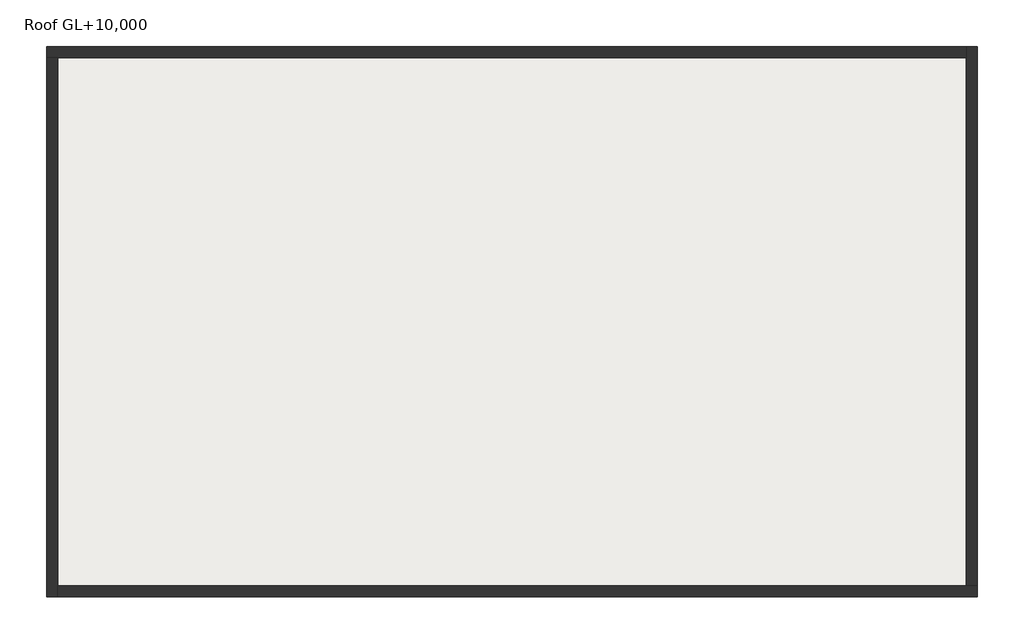
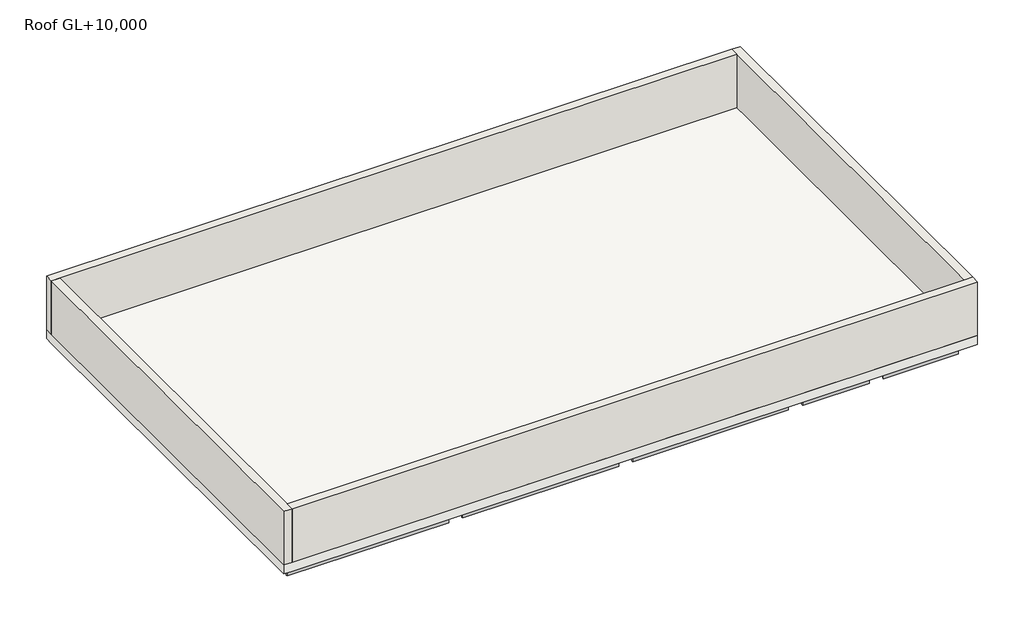
# One storey: 25 beams, 4 walls, 1 roof.
"""IFC4 building model written with IfcOpenShell, lengths in millimetres."""

from ifc_helpers import new_model, si_unit, frame, origin, place, context, project, spatial, polyline, outline, extrude, faceted_brep, element, save

model = new_model("IFC4")

# Units and contexts
model_context = context("Model", 3, world=origin())
ifc_project = project(units=[si_unit("LENGTHUNIT", "METRE", prefix="MILLI")], contexts=[model_context])

# Site, building, storey
site = spatial("IfcSite", under=ifc_project)
building = spatial("IfcBuilding", under=site)
storey = spatial("IfcBuildingStorey", under=building, Name="Roof GL+10,000", Elevation=10000.0)

# Beams
placement = place(None, origin())
element("IfcBeam", 1, ObjectType="RC Beam_Rectangular : 350 x 700mm", at=placement, inside=storey, context=model_context, shape_type="SweptSolid", body=[
    extrude(outline(polyline([(-18645.7273237, 1485.9763125), (-18595.7273237, 1485.9763125), (-18595.7273237, -4314.0236875), (-18645.7273237, -4314.0236875), (-18645.7273237, 1485.9763125)])), frame((0.0, 0.0, 9300.0), z_axis=(0.0, 0.0, 1.0), x_axis=(1.0, 0.0, 0.0)), (0.0, 0.0, 1.0), 367.0),
])
element("IfcBeam", 2, ObjectType="RC Beam_Rectangular : 350 x 700mm", at=placement, inside=storey, context=model_context, shape_type="SweptSolid", body=[
    extrude(outline(polyline([(-18645.7273237, 9185.9763125), (-18595.7273237, 9185.9763125), (-18595.7273237, 1985.9763125), (-18645.7273237, 1985.9763125), (-18645.7273237, 9185.9763125)])), frame((0.0, 0.0, 9300.0), z_axis=(0.0, 0.0, 1.0), x_axis=(1.0, 0.0, 0.0)), (0.0, 0.0, 1.0), 367.0),
])
element("IfcBeam", 3, ObjectType="RC Beam_Rectangular : 350 x 700mm", at=placement, inside=storey, context=model_context, shape_type="SweptSolid", body=[
    extrude(outline(polyline([(-12545.7273237, 1485.9763125), (-12520.7273237, 1485.9763125), (-12520.7273237, -4314.0236875), (-12545.7273237, -4314.0236875), (-12545.7273237, 1485.9763125)])), frame((0.0, 0.0, 9300.0), z_axis=(0.0, 0.0, 1.0), x_axis=(1.0, 0.0, 0.0)), (0.0, 0.0, 1.0), 367.0),
    extrude(outline(polyline([(-12870.7273237, 1485.9763125), (-12845.7273237, 1485.9763125), (-12845.7273237, -4314.0236875), (-12870.7273237, -4314.0236875), (-12870.7273237, 1485.9763125)])), frame((0.0, 0.0, 9300.0), z_axis=(0.0, 0.0, 1.0), x_axis=(1.0, 0.0, 0.0)), (0.0, 0.0, 1.0), 367.0),
])
element("IfcBeam", 4, ObjectType="RC Beam_Rectangular : 350 x 700mm", at=placement, inside=storey, context=model_context, shape_type="Brep", body=[
    faceted_brep([(-12520.7273237, 5725.9613486, 9667.0), (-12520.7273237, 5725.9613486, 9300.0), (-12520.7273237, 9185.9763125, 9300.0), (-12520.7273237, 9185.9763125, 9667.0), (-12545.7273237, 5725.9613486, 9300.0), (-12545.7273237, 9185.9763125, 9300.0), (-12545.7273237, 5725.9613486, 9667.0), (-12545.7273237, 9185.9763125, 9667.0)], [[[0, 1, 2, 3]], [[1, 4, 5, 2]], [[4, 6, 7, 5]], [[1, 0, 6, 4]], [[6, 0, 3, 7]], [[2, 5, 7, 3]]]),
    faceted_brep([(-12870.7273237, 9185.9763125, 9667.0), (-12870.7273237, 9185.9763125, 9300.0), (-12870.7273237, 1985.9763125, 9300.0), (-12870.7273237, 1985.9763125, 9667.0), (-12520.7273237, 5425.9613486, 9667.0), (-12545.7273237, 5425.9613486, 9667.0), (-12845.7273237, 5425.9613486, 9667.0), (-12845.7273237, 9185.9763125, 9667.0), (-12520.7273237, 1985.9763125, 9667.0), (-12845.7273237, 5425.9613486, 9300.0), (-12845.7273237, 9185.9763125, 9300.0), (-12520.7273237, 5425.9613486, 9300.0), (-12520.7273237, 1985.9763125, 9300.0)], [[[0, 1, 2, 3]], [[4, 5, 6, 7, 0, 3, 8]], [[6, 9, 10, 7]], [[9, 6, 5, 4, 11]], [[11, 4, 8, 12]], [[9, 11, 12, 2, 1, 10]], [[1, 0, 7, 10]], [[3, 2, 12, 8]]]),
])
element("IfcBeam", 5, ObjectType="RC Beam_Rectangular : 350 x 700mm", at=placement, inside=storey, context=model_context, shape_type="SweptSolid", body=[
    extrude(outline(polyline([(-6545.7273237, 1485.9763125), (-6520.7273237, 1485.9763125), (-6520.7273237, -4314.0236875), (-6545.7273237, -4314.0236875), (-6545.7273237, 1485.9763125)])), frame((0.0, 0.0, 9300.0), z_axis=(0.0, 0.0, 1.0), x_axis=(1.0, 0.0, 0.0)), (0.0, 0.0, 1.0), 367.0),
    extrude(outline(polyline([(-6870.7273237, 1485.9763125), (-6845.7273237, 1485.9763125), (-6845.7273237, -4314.0236875), (-6870.7273237, -4314.0236875), (-6870.7273237, 1485.9763125)])), frame((0.0, 0.0, 9300.0), z_axis=(0.0, 0.0, 1.0), x_axis=(1.0, 0.0, 0.0)), (0.0, 0.0, 1.0), 367.0),
])
element("IfcBeam", 6, ObjectType="RC Beam_Rectangular : 350 x 700mm", at=placement, inside=storey, context=model_context, shape_type="SweptSolid", body=[
    extrude(outline(polyline([(-6545.7273237, 9185.9763125), (-6520.7273237, 9185.9763125), (-6520.7273237, 1985.9763125), (-6545.7273237, 1985.9763125), (-6545.7273237, 9185.9763125)])), frame((0.0, 0.0, 9300.0), z_axis=(0.0, 0.0, 1.0), x_axis=(1.0, 0.0, 0.0)), (0.0, 0.0, 1.0), 367.0),
    extrude(outline(polyline([(-6845.7273237, 5725.9613486), (-6870.7273237, 5725.9613486), (-6870.7273237, 9185.9763125), (-6845.7273237, 9185.9763125), (-6845.7273237, 5725.9613486)])), frame((0.0, 0.0, 9300.0), z_axis=(0.0, 0.0, 1.0), x_axis=(1.0, 0.0, 0.0)), (0.0, 0.0, 1.0), 367.0),
    extrude(outline(polyline([(-6870.7273237, 5425.9613486), (-6845.7273237, 5425.9613486), (-6845.7273237, 1985.9763125), (-6870.7273237, 1985.9763125), (-6870.7273237, 5425.9613486)])), frame((0.0, 0.0, 9300.0), z_axis=(0.0, 0.0, 1.0), x_axis=(1.0, 0.0, 0.0)), (0.0, 0.0, 1.0), 367.0),
])
element("IfcBeam", 7, ObjectType="RC Beam_Rectangular : 350 x 700mm", at=placement, inside=storey, context=model_context, shape_type="SweptSolid", body=[
    extrude(outline(polyline([(-545.7273237, 1485.9763125), (-520.7273237, 1485.9763125), (-520.7273237, -4314.0236875), (-545.7273237, -4314.0236875), (-545.7273237, 1485.9763125)])), frame((0.0, 0.0, 9300.0), z_axis=(0.0, 0.0, 1.0), x_axis=(1.0, 0.0, 0.0)), (0.0, 0.0, 1.0), 367.0),
    extrude(outline(polyline([(-870.7273237, 1485.9763125), (-845.7273237, 1485.9763125), (-845.7273237, -4314.0236875), (-870.7273237, -4314.0236875), (-870.7273237, 1485.9763125)])), frame((0.0, 0.0, 9300.0), z_axis=(0.0, 0.0, 1.0), x_axis=(1.0, 0.0, 0.0)), (0.0, 0.0, 1.0), 367.0),
])
element("IfcBeam", 8, ObjectType="RC Beam_Rectangular : 350 x 700mm", at=placement, inside=storey, context=model_context, shape_type="SweptSolid", body=[
    extrude(outline(polyline([(-870.7273237, 9185.9763125), (-520.7273237, 9185.9763125), (-520.7273237, 1985.9763125), (-870.7273237, 1985.9763125), (-870.7273237, 9185.9763125)])), frame((0.0, 0.0, 9300.0), z_axis=(0.0, 0.0, 1.0), x_axis=(1.0, 0.0, 0.0)), (0.0, 0.0, 1.0), 367.0),
])
element("IfcBeam", 9, ObjectType="RC Beam_Rectangular : 350 x 700mm", at=placement, inside=storey, context=model_context, shape_type="SweptSolid", body=[
    extrude(outline(polyline([(5204.2726763, 1485.9763125), (5254.2726763, 1485.9763125), (5254.2726763, -4314.0236875), (5204.2726763, -4314.0236875), (5204.2726763, 1485.9763125)])), frame((0.0, 0.0, 9300.0), z_axis=(0.0, 0.0, 1.0), x_axis=(1.0, 0.0, 0.0)), (0.0, 0.0, 1.0), 367.0),
])
element("IfcBeam", 10, ObjectType="RC Beam_Rectangular : 350 x 700mm", at=placement, inside=storey, context=model_context, shape_type="SweptSolid", body=[
    extrude(outline(polyline([(5204.2726763, 9185.9763125), (5254.2726763, 9185.9763125), (5254.2726763, 1885.9763125), (5204.2726763, 1885.9763125), (5204.2726763, 9185.9763125)])), frame((0.0, 0.0, 9300.0), z_axis=(0.0, 0.0, 1.0), x_axis=(1.0, 0.0, 0.0)), (0.0, 0.0, 1.0), 367.0),
])
element("IfcBeam", 11, ObjectType="RC Beam_Rectangular : 350 x 700mm", at=placement, inside=storey, context=model_context, shape_type="SweptSolid", body=[
    extrude(outline(polyline([(-18445.7273237, 9335.9763125), (-18445.7273237, 9385.9763125), (-12945.7273237, 9385.9763125), (-12945.7273237, 9335.9763125), (-18445.7273237, 9335.9763125)])), frame((0.0, 0.0, 9300.0), z_axis=(0.0, 0.0, 1.0), x_axis=(1.0, 0.0, 0.0)), (0.0, 0.0, 1.0), 367.0),
])
element("IfcBeam", 12, ObjectType="RC Beam_Rectangular : 350 x 700mm", at=placement, inside=storey, context=model_context, shape_type="SweptSolid", body=[
    extrude(outline(polyline([(-12445.7273237, 9335.9763125), (-12445.7273237, 9385.9763125), (-6945.7273237, 9385.9763125), (-6945.7273237, 9335.9763125), (-12445.7273237, 9335.9763125)])), frame((0.0, 0.0, 9300.0), z_axis=(0.0, 0.0, 1.0), x_axis=(1.0, 0.0, 0.0)), (0.0, 0.0, 1.0), 367.0),
])
element("IfcBeam", 13, ObjectType="RC Beam_Rectangular : 350 x 700mm", at=placement, inside=storey, context=model_context, shape_type="SweptSolid", body=[
    extrude(outline(polyline([(-6445.7273237, 9335.9763125), (-6445.7273237, 9385.9763125), (-945.7273237, 9385.9763125), (-945.7273237, 9335.9763125), (-6445.7273237, 9335.9763125)])), frame((0.0, 0.0, 9300.0), z_axis=(0.0, 0.0, 1.0), x_axis=(1.0, 0.0, 0.0)), (0.0, 0.0, 1.0), 367.0),
])
element("IfcBeam", 14, ObjectType="RC Beam_Rectangular : 350 x 700mm", at=placement, inside=storey, context=model_context, shape_type="SweptSolid", body=[
    extrude(outline(polyline([(-445.7273237, 9385.9763125), (5254.2726763, 9385.9763125), (5254.2726763, 9335.9763125), (-445.7273237, 9335.9763125), (-445.7273237, 9385.9763125)])), frame((0.0, 0.0, 9300.0), z_axis=(0.0, 0.0, 1.0), x_axis=(1.0, 0.0, 0.0)), (0.0, 0.0, 1.0), 367.0),
])
element("IfcBeam", 15, ObjectType="RC Beam_Rectangular : 350 x 700mm", at=placement, inside=storey, context=model_context, shape_type="SweptSolid", body=[
    extrude(outline(polyline([(-18445.7273237, 1560.9763125), (-18445.7273237, 1585.9763125), (-12945.7273237, 1585.9763125), (-12945.7273237, 1560.9763125), (-18445.7273237, 1560.9763125)])), frame((0.0, 0.0, 9300.0), z_axis=(0.0, 0.0, 1.0), x_axis=(1.0, 0.0, 0.0)), (0.0, 0.0, 1.0), 367.0),
    extrude(outline(polyline([(-18445.7273237, 1885.9763125), (-18445.7273237, 1910.9763125), (-12945.7273237, 1910.9763125), (-12945.7273237, 1885.9763125), (-18445.7273237, 1885.9763125)])), frame((0.0, 0.0, 9300.0), z_axis=(0.0, 0.0, 1.0), x_axis=(1.0, 0.0, 0.0)), (0.0, 0.0, 1.0), 367.0),
])
element("IfcBeam", 16, ObjectType="RC Beam_Rectangular : 350 x 700mm", at=placement, inside=storey, context=model_context, shape_type="SweptSolid", body=[
    extrude(outline(polyline([(-12445.7273237, 1560.9763125), (-12445.7273237, 1585.9763125), (-6945.7273237, 1585.9763125), (-6945.7273237, 1560.9763125), (-12445.7273237, 1560.9763125)])), frame((0.0, 0.0, 9300.0), z_axis=(0.0, 0.0, 1.0), x_axis=(1.0, 0.0, 0.0)), (0.0, 0.0, 1.0), 367.0),
    extrude(outline(polyline([(-12445.7273237, 1885.9763125), (-12445.7273237, 1910.9763125), (-6945.7273237, 1910.9763125), (-6945.7273237, 1885.9763125), (-12445.7273237, 1885.9763125)])), frame((0.0, 0.0, 9300.0), z_axis=(0.0, 0.0, 1.0), x_axis=(1.0, 0.0, 0.0)), (0.0, 0.0, 1.0), 367.0),
])
element("IfcBeam", 17, ObjectType="RC Beam_Rectangular : 350 x 700mm", at=placement, inside=storey, context=model_context, shape_type="SweptSolid", body=[
    extrude(outline(polyline([(-6445.7273237, 1560.9763125), (-6445.7273237, 1585.9763125), (-945.7273237, 1585.9763125), (-945.7273237, 1560.9763125), (-6445.7273237, 1560.9763125)])), frame((0.0, 0.0, 9300.0), z_axis=(0.0, 0.0, 1.0), x_axis=(1.0, 0.0, 0.0)), (0.0, 0.0, 1.0), 367.0),
    extrude(outline(polyline([(-6445.7273237, 1885.9763125), (-6445.7273237, 1910.9763125), (-945.7273237, 1910.9763125), (-945.7273237, 1885.9763125), (-6445.7273237, 1885.9763125)])), frame((0.0, 0.0, 9300.0), z_axis=(0.0, 0.0, 1.0), x_axis=(1.0, 0.0, 0.0)), (0.0, 0.0, 1.0), 367.0),
])
element("IfcBeam", 18, ObjectType="RC Beam_Rectangular : 350 x 700mm", at=placement, inside=storey, context=model_context, shape_type="SweptSolid", body=[
    extrude(outline(polyline([(-445.7273237, 1560.9763125), (-445.7273237, 1585.9763125), (1904.2726763, 1585.9763125), (1904.2726763, 1560.9763125), (-445.7273237, 1560.9763125)])), frame((0.0, 0.0, 9300.0), z_axis=(0.0, 0.0, 1.0), x_axis=(1.0, 0.0, 0.0)), (0.0, 0.0, 1.0), 367.0),
    extrude(outline(polyline([(-445.7273237, 1885.9763125), (-445.7273237, 1910.9763125), (1904.2726763, 1910.9763125), (1904.2726763, 1885.9763125), (-445.7273237, 1885.9763125)])), frame((0.0, 0.0, 9300.0), z_axis=(0.0, 0.0, 1.0), x_axis=(1.0, 0.0, 0.0)), (0.0, 0.0, 1.0), 367.0),
])
element("IfcBeam", 19, ObjectType="RC Beam_Rectangular : 350 x 700mm", at=placement, inside=storey, context=model_context, shape_type="SweptSolid", body=[
    extrude(outline(polyline([(5054.2726763, 1585.9763125), (5054.2726763, 1560.9763125), (2404.2726763, 1560.9763125), (2404.2726763, 1585.9763125), (5054.2726763, 1585.9763125)])), frame((0.0, 0.0, 9300.0), z_axis=(0.0, 0.0, 1.0), x_axis=(1.0, 0.0, 0.0)), (0.0, 0.0, 1.0), 367.0),
    extrude(outline(polyline([(5054.2726763, 1910.9763125), (5054.2726763, 1885.9763125), (2404.2726763, 1885.9763125), (2404.2726763, 1910.9763125), (5054.2726763, 1910.9763125)])), frame((0.0, 0.0, 9300.0), z_axis=(0.0, 0.0, 1.0), x_axis=(1.0, 0.0, 0.0)), (0.0, 0.0, 1.0), 367.0),
])
element("IfcBeam", 20, ObjectType="RC Beam_Rectangular : 350 x 700mm", at=placement, inside=storey, context=model_context, shape_type="SweptSolid", body=[
    extrude(outline(polyline([(-12945.7273237, -4514.0236875), (-18645.7273237, -4514.0236875), (-18645.7273237, -4464.0236875), (-12945.7273237, -4464.0236875), (-12945.7273237, -4514.0236875)])), frame((0.0, 0.0, 9300.0), z_axis=(0.0, 0.0, 1.0), x_axis=(1.0, 0.0, 0.0)), (0.0, 0.0, 1.0), 367.0),
])
element("IfcBeam", 21, ObjectType="RC Beam_Rectangular : 350 x 700mm", at=placement, inside=storey, context=model_context, shape_type="SweptSolid", body=[
    extrude(outline(polyline([(-12445.7273237, -4514.0236875), (-12445.7273237, -4464.0236875), (-6945.7273237, -4464.0236875), (-6945.7273237, -4514.0236875), (-12445.7273237, -4514.0236875)])), frame((0.0, 0.0, 9300.0), z_axis=(0.0, 0.0, 1.0), x_axis=(1.0, 0.0, 0.0)), (0.0, 0.0, 1.0), 367.0),
])
element("IfcBeam", 22, ObjectType="RC Beam_Rectangular : 350 x 700mm", at=placement, inside=storey, context=model_context, shape_type="SweptSolid", body=[
    extrude(outline(polyline([(-6445.7273237, -4514.0236875), (-6445.7273237, -4464.0236875), (-945.7273237, -4464.0236875), (-945.7273237, -4514.0236875), (-6445.7273237, -4514.0236875)])), frame((0.0, 0.0, 9300.0), z_axis=(0.0, 0.0, 1.0), x_axis=(1.0, 0.0, 0.0)), (0.0, 0.0, 1.0), 367.0),
])
element("IfcBeam", 23, ObjectType="RC Beam_Rectangular : 350 x 700mm", at=placement, inside=storey, context=model_context, shape_type="SweptSolid", body=[
    extrude(outline(polyline([(-445.7273237, -4514.0236875), (-445.7273237, -4464.0236875), (1904.2726763, -4464.0236875), (1904.2726763, -4514.0236875), (-445.7273237, -4514.0236875)])), frame((0.0, 0.0, 9300.0), z_axis=(0.0, 0.0, 1.0), x_axis=(1.0, 0.0, 0.0)), (0.0, 0.0, 1.0), 367.0),
])
element("IfcBeam", 24, ObjectType="RC Beam_Rectangular : 350 x 700mm", at=placement, inside=storey, context=model_context, shape_type="SweptSolid", body=[
    extrude(outline(polyline([(5054.2726763, -4464.0236875), (5054.2726763, -4514.0236875), (2404.2726763, -4514.0236875), (2404.2726763, -4464.0236875), (5054.2726763, -4464.0236875)])), frame((0.0, 0.0, 9300.0), z_axis=(0.0, 0.0, 1.0), x_axis=(1.0, 0.0, 0.0)), (0.0, 0.0, 1.0), 367.0),
])
element("IfcBeam", 25, ObjectType="RC Beam_Rectangular : 350 x 700mm", at=placement, inside=storey, context=model_context, shape_type="SweptSolid", body=[
    extrude(outline(polyline([(2304.2726763, 1485.9763125), (2329.2726763, 1485.9763125), (2329.2726763, -4314.0236875), (2304.2726763, -4314.0236875), (2304.2726763, 1485.9763125)])), frame((0.0, 0.0, 9300.0), z_axis=(0.0, 0.0, 1.0), x_axis=(1.0, 0.0, 0.0)), (0.0, 0.0, 1.0), 367.0),
    extrude(outline(polyline([(1979.2726763, 1485.9763125), (2004.2726763, 1485.9763125), (2004.2726763, -4314.0236875), (1979.2726763, -4314.0236875), (1979.2726763, 1485.9763125)])), frame((0.0, 0.0, 9300.0), z_axis=(0.0, 0.0, 1.0), x_axis=(1.0, 0.0, 0.0)), (0.0, 0.0, 1.0), 367.0),
])

# Roof
element("IfcRoof", 26, ObjectType="H_RF_AMRF_Membrane_Insulation_Protection", at=placement, inside=storey, context=model_context, shape_type="Brep", body=[
    faceted_brep([(5554.2726763, 9685.9763125, 9667.0), (5554.2726763, -4514.0236875, 9667.0), (5554.2726763, -4814.0236875, 9667.0), (-18645.7273237, -4814.0236875, 9667.0), (-18945.7273237, -4814.0236875, 9667.0), (-18945.7273237, 9385.9763125, 9667.0), (-18945.7273237, 9685.9763125, 9667.0), (5254.2726763, 9685.9763125, 9667.0), (5554.2726763, -4814.0236875, 10000.0), (5554.2726763, 9685.9763125, 10000.0), (-18945.7273237, 9685.9763125, 10000.0), (-18945.7273237, -4814.0236875, 10000.0)], [[[0, 1, 2, 3, 4, 5, 6, 7]], [[8, 9, 10, 11]], [[9, 8, 2, 1, 0]], [[10, 9, 0, 7, 6]], [[11, 10, 6, 5, 4]], [[8, 11, 4, 3, 2]]]),
])

# Walls
element("IfcWall", 27, ObjectType="일반 - 300mm", at=placement, inside=storey, context=model_context, shape_type="Brep", body=[
    faceted_brep([(-18945.7273237, 9385.9763125, 10000.0), (-18645.7273237, 9385.9763125, 10000.0), (5254.2726763, 9385.9763125, 10000.0), (5254.2726763, 9385.9763125, 12000.0), (-18645.7273237, 9385.9763125, 12000.0), (-18945.7273237, 9385.9763125, 12000.0), (-18945.7273237, 9685.9763125, 10000.0), (-18945.7273237, 9685.9763125, 12000.0), (5254.2726763, 9685.9763125, 12000.0), (5254.2726763, 9685.9763125, 10000.0)], [[[0, 1, 2, 3, 4, 5]], [[6, 7, 8, 9]], [[2, 1, 0, 6, 9]], [[5, 4, 3, 8, 7]], [[0, 5, 7, 6]], [[3, 2, 9, 8]]]),
])
element("IfcWall", 28, ObjectType="일반 - 300mm", at=placement, inside=storey, context=model_context, shape_type="Brep", body=[
    faceted_brep([(-18645.7273237, -4814.0236875, 10000.0), (-18645.7273237, -4514.0236875, 10000.0), (-18645.7273237, 9385.9763125, 10000.0), (-18645.7273237, 9385.9763125, 12000.0), (-18645.7273237, -4514.0236875, 12000.0), (-18645.7273237, -4814.0236875, 12000.0), (-18945.7273237, -4814.0236875, 10000.0), (-18945.7273237, -4814.0236875, 12000.0), (-18945.7273237, 9385.9763125, 12000.0), (-18945.7273237, 9385.9763125, 10000.0)], [[[0, 1, 2, 3, 4, 5]], [[6, 7, 8, 9]], [[2, 1, 0, 6, 9]], [[5, 4, 3, 8, 7]], [[0, 5, 7, 6]], [[3, 2, 9, 8]]]),
])
element("IfcWall", 29, ObjectType="일반 - 300mm", at=placement, inside=storey, context=model_context, shape_type="Brep", body=[
    faceted_brep([(5554.2726763, -4514.0236875, 10000.0), (5254.2726763, -4514.0236875, 10000.0), (-18645.7273237, -4514.0236875, 10000.0), (-18645.7273237, -4514.0236875, 12000.0), (5254.2726763, -4514.0236875, 12000.0), (5554.2726763, -4514.0236875, 12000.0), (5554.2726763, -4814.0236875, 10000.0), (5554.2726763, -4814.0236875, 12000.0), (-18645.7273237, -4814.0236875, 12000.0), (-18645.7273237, -4814.0236875, 10000.0)], [[[0, 1, 2, 3, 4, 5]], [[6, 7, 8, 9]], [[2, 1, 0, 6, 9]], [[5, 4, 3, 8, 7]], [[0, 5, 7, 6]], [[3, 2, 9, 8]]]),
])
element("IfcWall", 30, ObjectType="일반 - 300mm", at=placement, inside=storey, context=model_context, shape_type="Brep", body=[
    faceted_brep([(5254.2726763, 9685.9763125, 10000.0), (5254.2726763, 9385.9763125, 10000.0), (5254.2726763, -4514.0236875, 10000.0), (5254.2726763, -4514.0236875, 12000.0), (5254.2726763, 9385.9763125, 12000.0), (5254.2726763, 9685.9763125, 12000.0), (5554.2726763, 9685.9763125, 10000.0), (5554.2726763, 9685.9763125, 12000.0), (5554.2726763, -4514.0236875, 12000.0), (5554.2726763, -4514.0236875, 10000.0)], [[[0, 1, 2, 3, 4, 5]], [[6, 7, 8, 9]], [[2, 1, 0, 6, 9]], [[5, 4, 3, 8, 7]], [[0, 5, 7, 6]], [[3, 2, 9, 8]]]),
])

save(model, "model.ifc")

# Revit data of these elements
# Type "RC Beam_Rectangular : 350 x 700mm"
#   Length [instance default] = 1524 mm
#   b = 350 mm
#   h = 700 mm
#   Structural Material [instance default] = 콘크리트, 현장타설 회색
#   Assembly Code = ""
# Type "H_RF_AMRF_Membrane_Insulation_Protection"
#   Layers, outside or top first: 38 mm "루핑, 타일" (function 4); 50 mm "고형 단열재" (function 3); 20 mm "아스팔트, 역청" (function 3); 0 mm "루핑 펠트" (function 100); 50 mm "콘크리트, 모래/시멘트 스크리드" (function 2); 175 mm "콘크리트, 현장치기" (function 1)
# Type "일반 - 300mm"
#   Layers, outside or top first: 300 mm no material (function 1)
# Elements 1, 2, 3, 4, 5, 6, 7, 8, 9, 10, 11, 12, 13, 14, 15, 16, 17, 18, 19, 20, 21, 22, 23, 24, 25 (IfcBeam, "RC Beam_Rectangular : 350 x 700mm")
#   Structural Material = 콘크리트, 현장타설 회색
#   Phase Created = 신축
#   Materials on its faces: "콘크리트, 현장타설 회색"
# Element 26 (IfcRoof, "H_RF_AMRF_Membrane_Insulation_Protection")
#   built-in parameter 1001705 = 32.8084 (stored number, unit not read)
#   built-in parameter 1001701 = -1.09252 (stored number, unit not read)
#   built-in parameter 1001710 = 33615
#   Phase Created = 신축
#   Materials on its faces: "콘크리트, 현장치기", "루핑, 타일"
# Elements 27, 28, 29, 30 (IfcWall, "일반 - 300mm")
#   Comments = ""
#   Top Offset = 0 mm
#   Base Offset = 0 mm
#   Unconnected Height = 2000 mm
#   wall height = 2000 mm
#   Phase Created = 신축
#   Base Constraint = Roof GL+10,000
#   Materials on its faces: "기본 벽"
# Materials
#   "콘크리트, 현장타설 회색": class "콘크리트", colour RGB 192 192 192, transparency 0, Description = "현장타설 콘크리트", Cost = 0
#   "루핑, 타일": class "금속", colour RGB 127 127 127, transparency 0, Description = "점토 루핑 타일", Cost = 0
#   "고형 단열재": class "일반", colour RGB 127 127 127, transparency 0, Description = "강체 폼 단열판", Cost = 0
#   "아스팔트, 역청": class "일반", colour RGB 155 155 155, transparency 0, Description = "역청 지붕 재료", Cost = 0
#   "루핑 펠트": class "일반", colour RGB 127 127 127, transparency 0, Description = "아스팔트 펠트", Cost = 0
#   "콘크리트, 모래/시멘트 스크리드": class "콘크리트", colour RGB 127 127 127, transparency 0, Description = "콘크리트 슬래브 덧침", Cost = 0
#   "콘크리트, 현장치기": class "콘크리트", colour RGB 192 192 192, transparency 0, Description = "물리적 재료", Cost = 0
#   "기본 벽": class "다양한", colour RGB 128 128 128, transparency 0, Cost = 0
